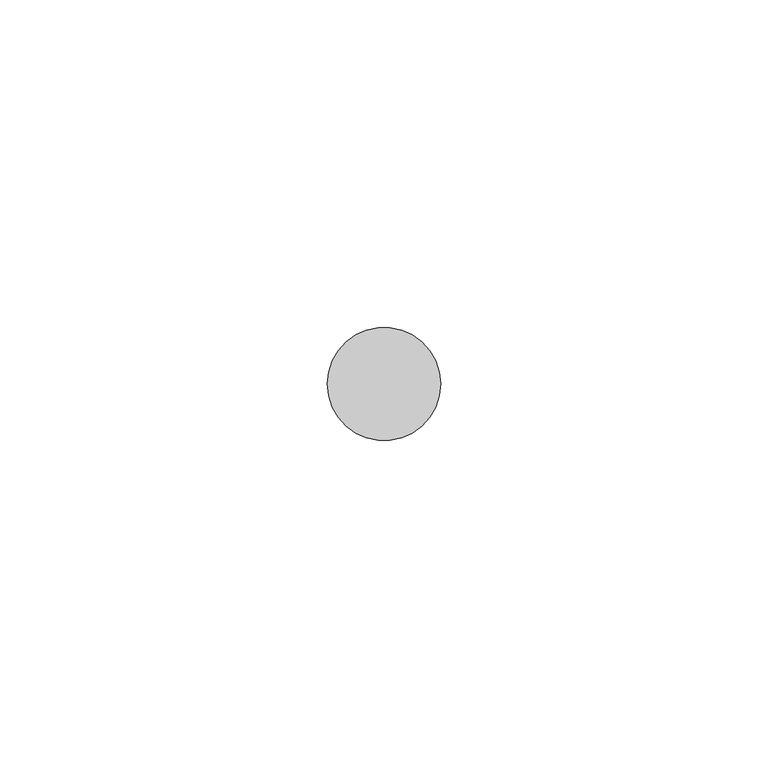
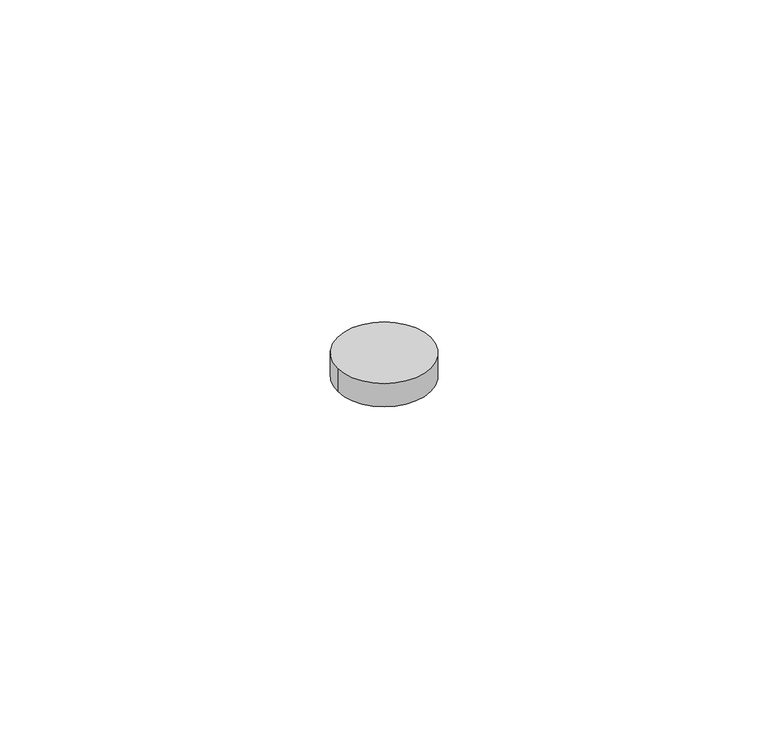
"""IFC4 building model written with IfcOpenShell, lengths in millimetres: proxy geometry, Hinge Pin Keeper3 : Hinge Pin Keeper."""

import ifcopenshell
import ifcopenshell.guid

model = None  # the IFC model being written
_history = None  # IfcOwnerHistory: only IFC2X3 demands one
_inside = {}  # id of a spatial element -> (the spatial element, [elements in it])
_under = {}  # id of a project, library or spatial element -> (it, [spatial elements below it])
_declared = {}  # id of a project -> (the project, [libraries it declares])
_typed = {}  # id of a type object -> (the type object, [elements of that type])
_made_of = {}  # id of a material, layer set ... -> (it, [elements and type objects made of it])


def new_model(schema):
    """Start an empty IFC model of exactly this schema.

    Asked for "IFC4X3", IfcOpenShell would pick the latest addendum, in which some entities
    have other attributes; the version numbers below select the first issue.
    IFC2X3 requires an IfcOwnerHistory on every rooted entity: one is made here for all.
    """
    global model, _history
    if schema == "IFC4X3":
        model = ifcopenshell.file(schema_version=(4, 3, 0, 0))
    else:
        model = ifcopenshell.file(schema=schema)
    _inside.clear()
    _under.clear()
    _declared.clear()
    _typed.clear()
    _made_of.clear()
    _history = None
    if model.schema == "IFC2X3":
        org = make("IfcOrganization", Name="unknown")
        user = make(
            "IfcPersonAndOrganization",
            ThePerson=make("IfcPerson", FamilyName="unknown"),
            TheOrganization=org,
        )
        app = make(
            "IfcApplication",
            ApplicationDeveloper=org,
            Version="unknown",
            ApplicationFullName="unknown",
            ApplicationIdentifier="unknown",
        )
        _history = make(
            "IfcOwnerHistory",
            OwningUser=user,
            OwningApplication=app,
            ChangeAction="ADDED",
            CreationDate=0,
        )
    return model


def make(cls, **values):
    """One entity of the class cls with the attributes given. An attribute that is None is left unset."""
    return model.create_entity(
        cls, **{name: value for name, value in values.items() if value is not None}
    )


def rooted(cls, **values):
    """An entity with a GlobalId (a new one), such as an element, a storey or a relation."""
    return make(cls, GlobalId=ifcopenshell.guid.new(), OwnerHistory=_history, **values)


def si_unit(unit_type, name, prefix=None):
    """IfcSIUnit, for example si_unit("LENGTHUNIT", "METRE", prefix="MILLI")."""
    return make("IfcSIUnit", UnitType=unit_type, Prefix=prefix, Name=name)


def assignment(units):
    """IfcUnitAssignment: the units of a project."""
    return None if units is None else make("IfcUnitAssignment", Units=units)


def point(xyz):
    """IfcCartesianPoint."""
    return None if xyz is None else make("IfcCartesianPoint", Coordinates=xyz)


def direction(xyz):
    """IfcDirection."""
    return None if xyz is None else make("IfcDirection", DirectionRatios=xyz)


def frame(location, z_axis=None, x_axis=None):
    """IfcAxis2Placement3D, a coordinate frame: its origin and axes. An axis left out is left unset."""
    return make(
        "IfcAxis2Placement3D",
        Location=point(location),
        Axis=direction(z_axis),
        RefDirection=direction(x_axis),
    )


def frame_2d(location, x_axis=None):
    """IfcAxis2Placement2D, a coordinate frame in the plane: its origin and x axis."""
    return make(
        "IfcAxis2Placement2D", Location=point(location), RefDirection=direction(x_axis)
    )


def origin():
    """The frame at (0, 0, 0) with its axes left unset."""
    return frame((0.0, 0.0, 0.0))


def place(relative_to, where):
    """IfcLocalPlacement: puts the frame where relative to a parent placement (None: the world)."""
    return make(
        "IfcLocalPlacement", PlacementRelTo=relative_to, RelativePlacement=where
    )


def context(
    kind, dimensions, precision=None, world=None, true_north=None, identifier=None
):
    """IfcGeometricRepresentationContext, for example the 3D "Model" context."""
    return make(
        "IfcGeometricRepresentationContext",
        ContextIdentifier=identifier,
        ContextType=kind,
        CoordinateSpaceDimension=dimensions,
        Precision=precision,
        WorldCoordinateSystem=world,
        TrueNorth=true_north,
    )


def project(units=None, contexts=None):
    """IfcProject with its units and contexts."""
    return rooted(
        "IfcProject",
        Name="project",
        RepresentationContexts=contexts,
        UnitsInContext=assignment(units),
    )


def spatial(cls, under=None, at=None, **own):
    """A site, building, storey or space (cls), placed at a placement, below another one or the project."""
    s = rooted(cls, ObjectPlacement=at, **own)
    if under is not None:
        _under.setdefault(under.id(), (under, []))[1].append(s)
    return s


def circle_curve(where, radius):
    """IfcCircle in the frame where."""
    return make("IfcCircle", Position=where, Radius=radius)


def trimmed(basis, trim1, trim2, sense, master):
    """IfcTrimmedCurve: the piece of a basis curve between two trims."""
    return make(
        "IfcTrimmedCurve",
        BasisCurve=basis,
        Trim1=trim1,
        Trim2=trim2,
        SenseAgreement=sense,
        MasterRepresentation=master,
    )


def segment(curve, same_sense, transition):
    """IfcCompositeCurveSegment."""
    return make(
        "IfcCompositeCurveSegment",
        Transition=transition,
        SameSense=same_sense,
        ParentCurve=curve,
    )


def composite_curve(segments, self_intersect=None):
    """IfcCompositeCurve: segments joined end to end."""
    return make("IfcCompositeCurve", Segments=segments, SelfIntersect=self_intersect)


def outline(outer, holes=None, kind="AREA"):
    """IfcArbitraryClosedProfileDef: a profile drawn as a closed curve; with holes, ...WithVoids."""
    if holes is None:
        return make("IfcArbitraryClosedProfileDef", ProfileType=kind, OuterCurve=outer)
    return make(
        "IfcArbitraryProfileDefWithVoids",
        ProfileType=kind,
        OuterCurve=outer,
        InnerCurves=holes,
    )


def extrude(swept, where, along, depth):
    """IfcExtrudedAreaSolid: the profile swept, set in the frame where, extruded along a direction by depth."""
    return make(
        "IfcExtrudedAreaSolid",
        SweptArea=swept,
        Position=where,
        ExtrudedDirection=direction(along),
        Depth=depth,
    )


def shape(context_of_items, identifier, shape_type, items):
    """IfcShapeRepresentation: the items that make up one representation, for example the "Body"."""
    return make(
        "IfcShapeRepresentation",
        ContextOfItems=context_of_items,
        RepresentationIdentifier=identifier,
        RepresentationType=shape_type,
        Items=items,
    )


def source(mapping_origin, context_of_items, identifier, shape_type, items):
    """IfcRepresentationMap: a shape defined once, which mapped items show again and again."""
    return make(
        "IfcRepresentationMap",
        MappingOrigin=mapping_origin,
        MappedRepresentation=shape(context_of_items, identifier, shape_type, items),
    )


def transform(
    local_origin,
    x_axis=None,
    y_axis=None,
    z_axis=None,
    scale=None,
    scale2=None,
    scale3=None,
    uniform=True,
):
    """IfcCartesianTransformationOperator3D, or its non-uniform kind. x_axis, y_axis, z_axis: its Axis1, 2, 3."""
    if uniform:
        return make(
            "IfcCartesianTransformationOperator3D",
            Axis1=direction(x_axis),
            Axis2=direction(y_axis),
            LocalOrigin=point(local_origin),
            Scale=scale,
            Axis3=direction(z_axis),
        )
    return make(
        "IfcCartesianTransformationOperator3DnonUniform",
        Axis1=direction(x_axis),
        Axis2=direction(y_axis),
        LocalOrigin=point(local_origin),
        Scale=scale,
        Axis3=direction(z_axis),
        Scale2=scale2,
        Scale3=scale3,
    )


def mapped(mapping_source, mapping_target):
    """IfcMappedItem: shows the shape of a source again, moved by a transform."""
    return make(
        "IfcMappedItem", MappingSource=mapping_source, MappingTarget=mapping_target
    )


def made_of(thing, what):
    """Note that an element or type object is made of a material, layer set ...; save() writes the relation."""
    if what is not None:
        _made_of.setdefault(what.id(), (what, []))[1].append(thing)
    return thing


def element(
    cls,
    number,
    at=None,
    inside=None,
    cuts=None,
    type_object=None,
    material=None,
    context=None,
    identifier="Body",
    shape_type=None,
    held_by="IfcProductDefinitionShape",
    body=None,
    shapes=None,
    **own,
):
    """One element of the class cls, such as IfcWall. Its Tag is "e" and its number.

    at: its placement. inside: the storey or other place that contains it. cuts: it is an
    opening in that element (IfcRelVoidsElement). A single representation is given by context,
    identifier, shape_type and body (its items); several are given by shapes. held_by: the class
    of the entity that holds the representations. save() writes the other relations.
    """
    e = rooted(cls, Tag="e%d" % number, ObjectPlacement=at, **own)
    if body is not None:
        shapes = [shape(context, identifier, shape_type, body)]
    if shapes is not None:
        e.Representation = make(held_by, Representations=shapes)
    if inside is not None:
        _inside.setdefault(inside.id(), (inside, []))[1].append(e)
    if cuts is not None:
        rooted(
            "IfcRelVoidsElement", RelatingBuildingElement=cuts, RelatedOpeningElement=e
        )
    if type_object is not None:
        _typed.setdefault(type_object.id(), (type_object, []))[1].append(e)
    return made_of(e, material)


def aggregate(whole, parts):
    """IfcRelAggregates: a whole, such as a stair, and the parts it consists of."""
    return rooted("IfcRelAggregates", RelatingObject=whole, RelatedObjects=parts)


def save(model, path):
    """Write the relations noted so far, then the file.

    IfcRelAggregates (storeys below a building ...), IfcRelContainedInSpatialStructure (elements
    in a storey), IfcRelDefinesByType, IfcRelAssociatesMaterial and IfcRelDeclares: one each for
    every whole, place, type object, material and project.
    """
    for whole, parts in _under.values():
        aggregate(whole, parts)
    for where, things in _inside.values():
        rooted(
            "IfcRelContainedInSpatialStructure",
            RelatedElements=things,
            RelatingStructure=where,
        )
    for kind, things in _typed.values():
        rooted("IfcRelDefinesByType", RelatedObjects=things, RelatingType=kind)
    for what, things in _made_of.values():
        rooted("IfcRelAssociatesMaterial", RelatedObjects=things, RelatingMaterial=what)
    for by, libraries in _declared.values():
        rooted("IfcRelDeclares", RelatingContext=by, RelatedDefinitions=libraries)
    model.write(path)


def generic_models_3964e635(model_context):
    return source(origin(), model_context, "Body", "SweptSolid", [
        extrude(outline(composite_curve([segment(trimmed(circle_curve(frame_2d((587319.1320739, -533984.6777841)), 8.6534625), [point((587310.4786114, -533984.6777841))], [point((587327.7855364, -533984.6777841))], False, "CARTESIAN"), True, "CONTINUOUS"), segment(trimmed(circle_curve(frame_2d((587319.1320739, -533984.6777841)), 8.6534625), [point((587327.7855364, -533984.6777841))], [point((587310.4786114, -533984.6777841))], False, "CARTESIAN"), True, "CONTINUOUS")], self_intersect=False)), frame((0.0, 0.0, 2084.5859375), z_axis=(0.0, 0.0, 1.0), x_axis=(1.0, 0.0, 0.0)), (0.0, 0.0, 1.0), 4.5640625),
    ])


if __name__ == "__main__":
    model = new_model("IFC4")
    model_context = context("Model", 3, world=origin())
    ifc_project = project(units=[si_unit("LENGTHUNIT", "METRE", prefix="MILLI")], contexts=[model_context])
    site = spatial("IfcSite", under=ifc_project)
    building = spatial("IfcBuilding", under=site)
    placement = place(None, origin())
    generic_models_shape = generic_models_3964e635(model_context)
    element("IfcBuildingElementProxy", 1, Name="Hinge Pin Keeper3 : Hinge Pin Keeper", ObjectType="Hinge Pin Keeper3 : Hinge Pin Keeper", at=placement, inside=building, context=model_context, shape_type="MappedRepresentation", body=[
        mapped(generic_models_shape, transform((0.0, 0.0, 0.0), x_axis=(1.0, 0.0, 0.0), y_axis=(0.0, 1.0, 0.0), z_axis=(0.0, 0.0, 1.0))),
    ])
    save(model, "model.ifc")

# Revit data of these elements
# Element 1 (IfcBuildingElementProxy, "Hinge Pin Keeper3 : Hinge Pin Keeper")
#   Materials on its faces: "6\"X6\" WELD-ON STL BUTT HINGE"
# Materials
#   "6\"X6\" WELD-ON STL BUTT HINGE": class "Metal", colour RGB 189 187 185, transparency 0, Description = "Carbon steel", Cost = 0
